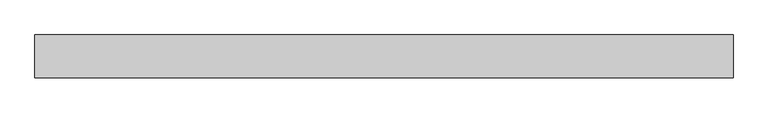
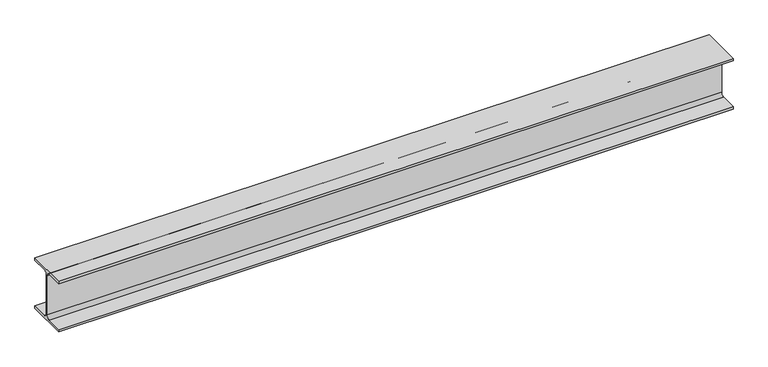
"""IFC4 building model written with IfcOpenShell, lengths in millimetres: beam geometry, 0912_Steel Framing_H-KSD3502 : H_SB_ASB_H-194x150x6x9."""

from ifc_helpers import new_model, si_unit, point, frame, frame_2d, origin, place, context, project, spatial, polyline, circle_curve, trimmed, segment, composite_curve, outline, extrude, source, transform, mapped, element, save


def beam_f1aeb8a8(model_context):
    return source(origin(), model_context, "Body", "SweptSolid", [
        extrude(outline(composite_curve([segment(polyline([(-75.0, -88.0), (-16.0, -88.0)]), True, "CONTINUOUS"), segment(trimmed(circle_curve(frame_2d((-16.0, -75.0)), 13.0), [point((-16.0, -88.0))], [point((-3.0, -75.0))], True, "CARTESIAN"), True, "CONTINUOUS"), segment(polyline([(-3.0, -75.0), (-3.0, 75.0)]), True, "CONTINUOUS"), segment(trimmed(circle_curve(frame_2d((-16.0, 75.0)), 13.0), [point((-3.0, 75.0))], [point((-16.0, 88.0))], True, "CARTESIAN"), True, "CONTINUOUS"), segment(polyline([(-16.0, 88.0), (-75.0, 88.0), (-75.0, 97.0), (75.0, 97.0), (75.0, 88.0), (16.0, 88.0)]), True, "CONTINUOUS"), segment(trimmed(circle_curve(frame_2d((16.0, 75.0)), 13.0), [point((16.0, 88.0))], [point((3.0, 75.0))], True, "CARTESIAN"), True, "CONTINUOUS"), segment(polyline([(3.0, 75.0), (3.0, -75.0)]), True, "CONTINUOUS"), segment(trimmed(circle_curve(frame_2d((16.0, -75.0)), 13.0), [point((3.0, -75.0))], [point((16.0, -88.0))], True, "CARTESIAN"), True, "CONTINUOUS"), segment(polyline([(16.0, -88.0), (75.0, -88.0), (75.0, -97.0), (-75.0, -97.0), (-75.0, -88.0)]), True, "CONTINUOUS")], self_intersect=False)), frame((-1200.0, 0.0, 0.0), z_axis=(1.0, 0.0, 0.0), x_axis=(0.0, 1.0, 0.0)), (0.0, 0.0, 1.0), 2448.0465428),
    ])


if __name__ == "__main__":
    model = new_model("IFC4")
    model_context = context("Model", 3, world=origin())
    ifc_project = project(units=[si_unit("LENGTHUNIT", "METRE", prefix="MILLI")], contexts=[model_context])
    site = spatial("IfcSite", under=ifc_project)
    building = spatial("IfcBuilding", under=site)
    placement = place(None, origin())
    beam_shape = beam_f1aeb8a8(model_context)
    element("IfcBeam", 1, ObjectType="0912_Steel Framing_H-KSD3502 : H_SB_ASB_H-194x150x6x9", at=placement, inside=building, context=model_context, shape_type="MappedRepresentation", body=[
        mapped(beam_shape, transform((0.0, 0.0, 0.0), x_axis=(1.0, 0.0, 0.0), y_axis=(0.0, 1.0, 0.0), z_axis=(0.0, 0.0, 1.0))),
    ])
    save(model, "model.ifc")

# Revit data of these elements
# Type "0912_Steel Framing_H-KSD3502 : H_SB_ASB_H-194x150x6x9"
#   H_WM Code_1 = "S01AA002-00001 | Main Steel Structure Fabrication Work | Shelter/Building | Medium Steel - Standard (90KG/M>Weight≥30KG/M) | Material: (   )"
#   H_WM Code_2 = "S03AA028-00001 | Main Steel Structure Erection Work | Shelter/Building | Medium Steel (90KG/M>Weight≥30KG/M) | Material: (   )"
#   H_WM Code_3 = "S01AA010-00001 | Main Steel Structure Fabrication Work | Shelter/Building | Steel Painting/Coating | for Non-Fireproofed Steel Surface, Surface Preparation, Primer, Second & Final Coat | Material: (   )"
#   H_Q'ty Cal Type Tag = "SB-Q2"
#   Width = 15.0 cm
#   Web Thickness = 0.6 cm
#   Web Fillet = 1.3 cm
#   Warping Constant = 43316.0 cm⁶
#   W = 0
#   Torsional Moment of Inertia = 8.622 cm⁴
#   Section Area = 39.01 cm²
#   Plastic Modulus weak axis = 104.0 cm³
#   Plastic Modulus strong axis = 309.0 cm³
#   Perimeter = 0.95 m²/m
#   Nominal Weight = 30.60 kgf/m
#   Moment of Inertia weak axis = 507.00 cm⁴
#   Moment of Inertia strong axis = 2690.00 cm⁴
#   Height = 19.4 cm
#   Flange Thickness = 0.9 cm
#   Elastic Modulus weak axis = 67.6 cm³
#   Elastic Modulus strong axis = 277.0 cm³
#   Centroid Vertical = 9.7 cm
#   Centroid Horizontal = 7.5 cm
#   Ix = 26900000
#   Length [instance default] = 1.5240 m
#   Zx = 309000
#   b = 0.1500 m
#   h = 0.1940 m
#   r = 0.0130 m
#   s = 0.0060 m
#   t = 0.0090 m
#   A = 0.003901 m²
#   Structural Material [instance default] = Steel, 45-345
#   Assembly Code = ""
# Element 1 (IfcBeam, "0912_Steel Framing_H-KSD3502 : H_SB_ASB_H-194x150x6x9")
#   Structural Material = none
# Materials
#   "Steel, 45-345": class "Metal", colour RGB 189 187 185, transparency 0, Description = "Steel 345 MPa", Cost = 0
